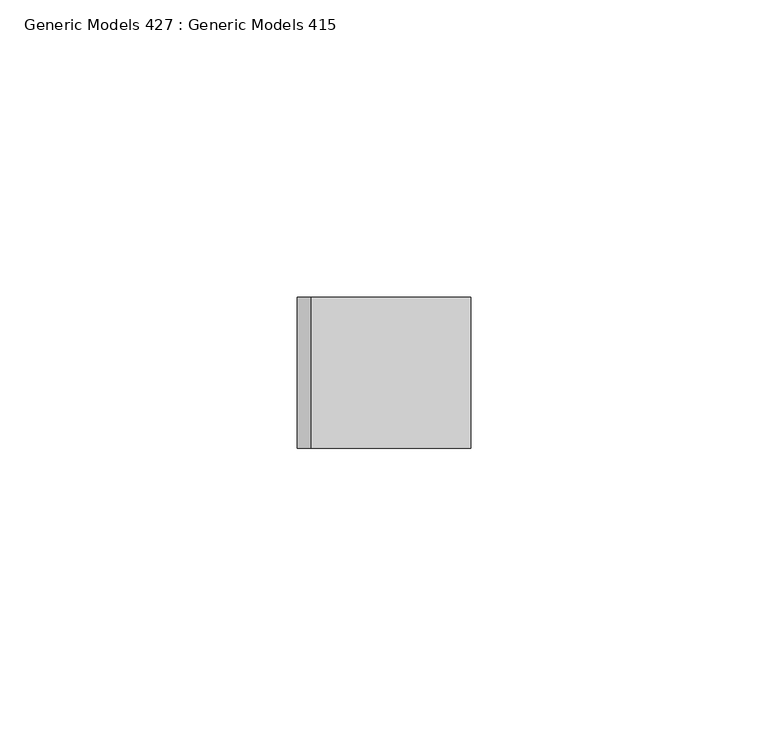
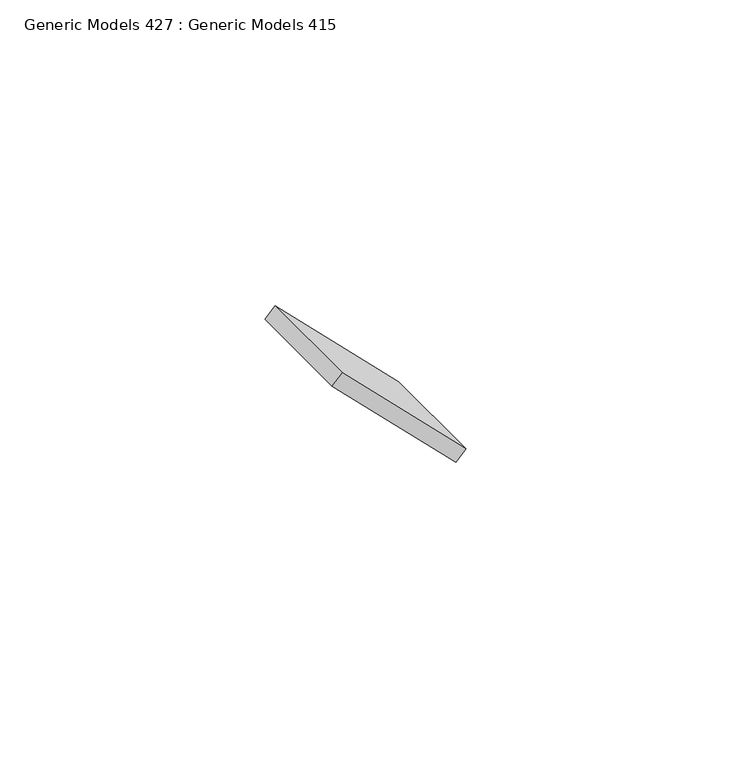
"""IFC4 building model written with IfcOpenShell, lengths in millimetres: proxy geometry, Generic Models 427 : Generic Models 415."""

from ifc_helpers import new_model, si_unit, frame, origin, place, context, project, spatial, polyline, outline, extrude, source, transform, mapped, element, save


def generic_models_427_generic_models_415_5fe5dea6(model_context):
    return source(origin(), model_context, "Body", "SweptSolid", [
        extrude(outline(polyline([(0.0, -38.1), (0.0, 0.0), (25.4, 0.0), (25.4, -38.1), (0.0, -38.1)])), frame((-6869.8996186, -4475.9863946, 128416.5002957), z_axis=(0.7071067811864907, 0.0, 0.7071067811866044), x_axis=(0.0, -1.0, 0.0)), (0.0, 0.0, 1.0), 3.175),
    ])


if __name__ == "__main__":
    model = new_model("IFC4")
    model_context = context("Model", 3, world=origin())
    ifc_project = project(units=[si_unit("LENGTHUNIT", "METRE", prefix="MILLI")], contexts=[model_context])
    site = spatial("IfcSite", under=ifc_project)
    building = spatial("IfcBuilding", under=site)
    placement = place(None, origin())
    generic_models_427_generic_models_415_shape = generic_models_427_generic_models_415_5fe5dea6(model_context)
    element("IfcBuildingElementProxy", 1, Name="Generic Models 427 : Generic Models 415", ObjectType="Generic Models 427 : Generic Models 415", at=placement, inside=building, context=model_context, shape_type="MappedRepresentation", body=[
        mapped(generic_models_427_generic_models_415_shape, transform((0.0, 0.0, 0.0), x_axis=(1.0, 0.0, 0.0), y_axis=(0.0, 1.0, 0.0), z_axis=(0.0, 0.0, 1.0))),
    ])
    save(model, "model.ifc")

# Revit data of these elements
# Element 1 (IfcBuildingElementProxy, "Generic Models 427 : Generic Models 415")
#   Materials on its faces: "_WELDED STEEL TABS FOR LOUVER ATTACHMENT"
# Materials
#   "_WELDED STEEL TABS FOR LOUVER ATTACHMENT": class "Metal", colour RGB 199 199 199, transparency 0, Description = "Structural steel 50ksi", Cost = 0
